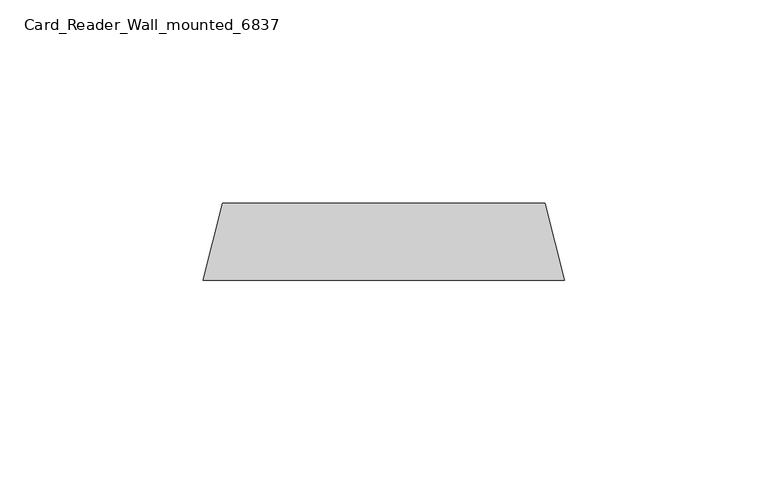
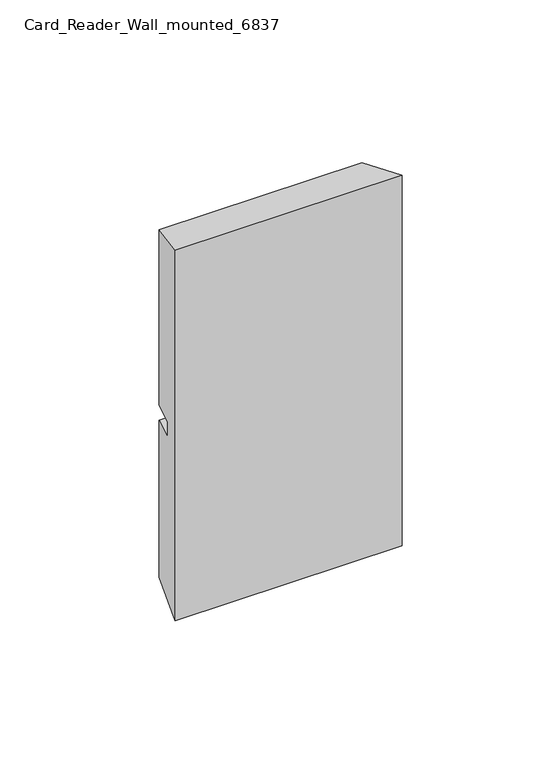
"""IFC4 building model written with IfcOpenShell, lengths in millimetres: proxy geometry, Card_Reader_Wall_mounted_6837 : swipe."""

from ifc_helpers import new_model, si_unit, origin, place, context, project, spatial, faceted_brep, source, transform, mapped, element, save


def card_reader_wall_mounted_6837_103fc86f(model_context):
    return source(origin(), model_context, "Body", "Brep", [
        faceted_brep([(20.6375, 93.9392764, 1265.2375), (100.0125, 93.9392764, 1265.2375), (100.0125, 93.9392764, 1192.6911313), (20.6375, 93.9392764, 1192.6911313), (100.0125, 93.9392764, 1121.2536313), (20.6375, 93.9392764, 1121.2536313), (20.6375, 93.9392764, 1186.3411313), (100.0125, 93.9392764, 1186.3411313), (15.875, 75.0, 1270.0), (15.875, 75.0, 1116.4911313), (104.775, 75.0, 1116.4911313), (104.775, 75.0, 1270.0), (102.4977808, 84.0559335, 1186.3411313), (102.4977808, 84.0559335, 1192.6911313), (18.1522192, 84.0559335, 1192.6911313), (18.1522192, 84.0559335, 1186.3411313)], [[[0, 1, 2, 3]], [[4, 5, 6, 7]], [[8, 9, 10, 11]], [[1, 0, 8, 11]], [[11, 10, 4, 7, 12, 13, 2, 1]], [[5, 4, 10, 9]], [[9, 8, 0, 3, 14, 15, 6, 5]], [[14, 13, 12, 15]], [[15, 12, 7, 6]], [[13, 14, 3, 2]]]),
    ])


if __name__ == "__main__":
    model = new_model("IFC4")
    model_context = context("Model", 3, world=origin())
    ifc_project = project(units=[si_unit("LENGTHUNIT", "METRE", prefix="MILLI")], contexts=[model_context])
    site = spatial("IfcSite", under=ifc_project)
    building = spatial("IfcBuilding", under=site)
    placement = place(None, origin())
    card_reader_wall_mounted_6837_shape = card_reader_wall_mounted_6837_103fc86f(model_context)
    element("IfcBuildingElementProxy", 1, Name="Card_Reader_Wall_mounted_6837 : swipe", ObjectType="Card_Reader_Wall_mounted_6837 : swipe", at=placement, inside=building, context=model_context, shape_type="MappedRepresentation", body=[
        mapped(card_reader_wall_mounted_6837_shape, transform((0.0, 0.0, 0.0), x_axis=(1.0, 0.0, 0.0), y_axis=(0.0, 1.0, 0.0), z_axis=(0.0, 0.0, 1.0))),
    ])
    save(model, "model.ifc")

# Revit data of these elements
# Type "Card_Reader_Wall_mounted_6837 : swipe"
#   COBie.Type.CreatedBy = "design@eagle.com"
#   COBie.Type.CreatedOn = "2016-09-13T05:47:35"
#   COBie.Type.Name = "Security Devices_Card_Reader_Wall_mounted_6837_swipe"
#   COBie.Type.Category = "23-85 30 11 : Access Controls"
#   COBie.Type.Description = ""
#   COBie.Type.Manufacturer = ""
#   COBie.Type.ModelNumber = ""
#   COBie.Type.ReplacementCost = 0
#   Width = 69.85 mm
#   Placement Height = 304.8 mm
#   Height = 114.3 mm
#   COBie.Type = yes
#   Material = Plastic - Black
#   Assembly Code = ""
# Element 1 (IfcBuildingElementProxy, "Card_Reader_Wall_mounted_6837 : swipe")
#   Materials on its faces: "Plastic - Black"
# Materials
#   "Plastic - Black": class "Plastic", colour RGB 0 0 0, transparency 0
